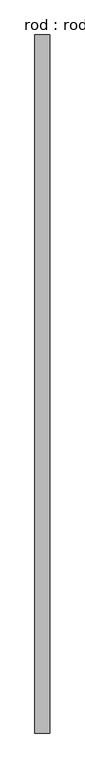
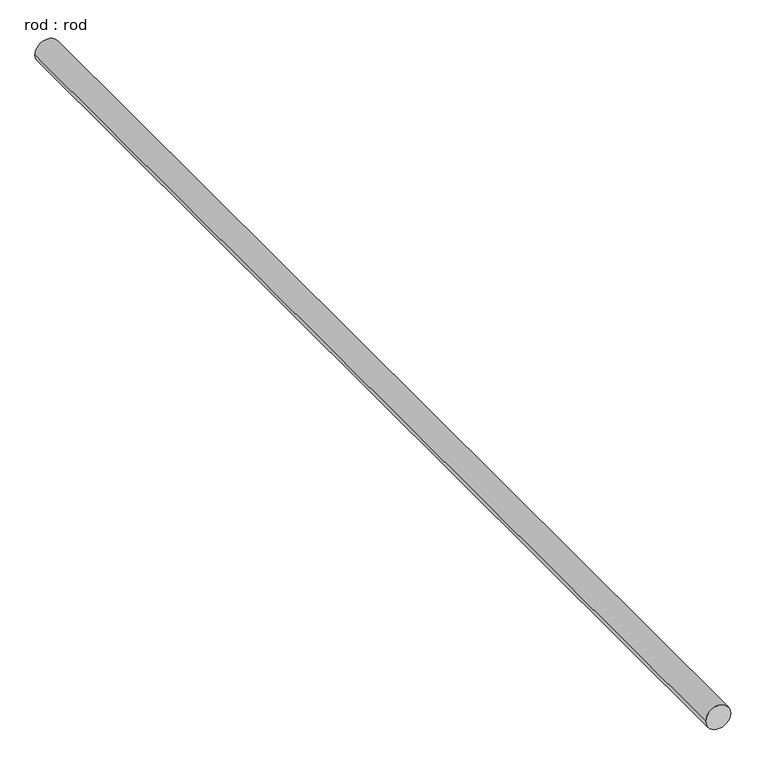
"""IFC4 building model written with IfcOpenShell, lengths in millimetres: proxy geometry, rod : rod."""

from ifc_helpers import new_model, si_unit, point, frame, frame_2d, origin, place, context, project, spatial, circle_curve, trimmed, segment, composite_curve, outline, extrude, source, transform, mapped, element, save


def rod_rod_83d7496f(model_context):
    return source(origin(), model_context, "Body", "SweptSolid", [
        extrude(outline(composite_curve([segment(trimmed(circle_curve(frame_2d((0.0108462, 0.0)), 200.0), [point((0.0108462, 200.0))], [point((0.0108462, -200.0))], False, "CARTESIAN"), True, "CONTINUOUS"), segment(trimmed(circle_curve(frame_2d((0.0108462, 0.0)), 200.0), [point((0.0108462, -200.0))], [point((0.0108462, 200.0))], False, "CARTESIAN"), True, "CONTINUOUS")], self_intersect=False)), frame((0.0, -5266.1829243, 0.0), z_axis=(0.0, 1.0, 0.0), x_axis=(0.0, 0.0, 1.0)), (0.0, 0.0, 1.0), 18717.8230793),
    ])


if __name__ == "__main__":
    model = new_model("IFC4")
    model_context = context("Model", 3, world=origin())
    ifc_project = project(units=[si_unit("LENGTHUNIT", "METRE", prefix="MILLI")], contexts=[model_context])
    site = spatial("IfcSite", under=ifc_project)
    building = spatial("IfcBuilding", under=site)
    placement = place(None, origin())
    rod_rod_shape = rod_rod_83d7496f(model_context)
    element("IfcBuildingElementProxy", 1, Name="rod : rod", ObjectType="rod : rod", at=placement, inside=building, context=model_context, shape_type="MappedRepresentation", body=[
        mapped(rod_rod_shape, transform((0.0, 0.0, 0.0), x_axis=(1.0, 0.0, 0.0), y_axis=(0.0, 1.0, 0.0), z_axis=(0.0, 0.0, 1.0))),
    ])
    save(model, "model.ifc")

# Revit data of these elements
# Type "rod : rod"
#   Default Elevation = 0
